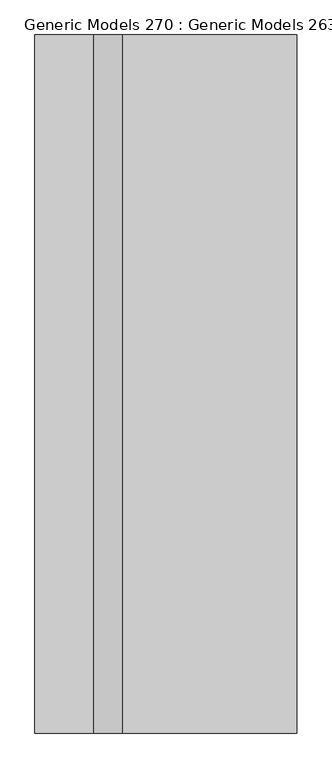
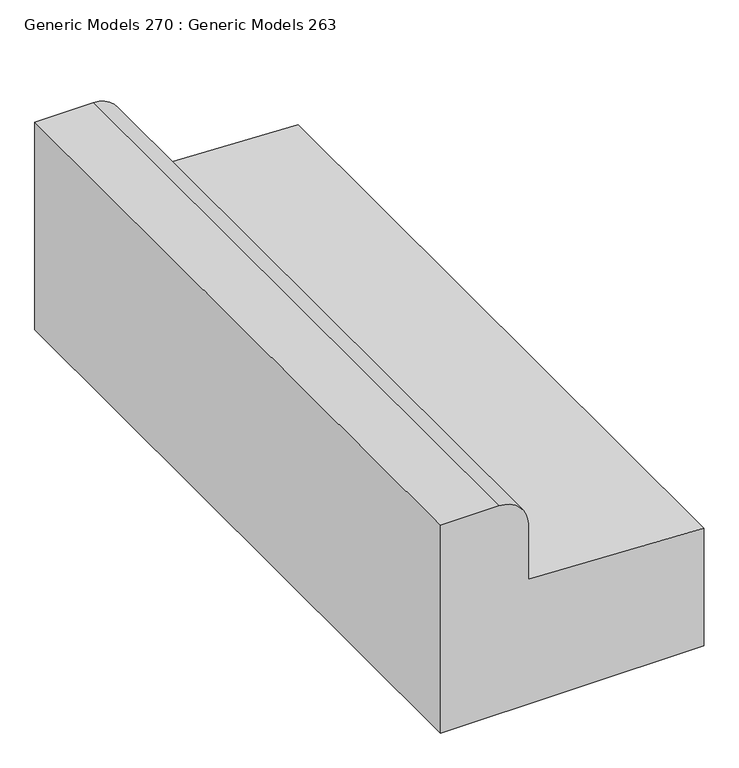
"""IFC4 building model written with IfcOpenShell, lengths in millimetres: proxy geometry, Generic Models 270 : Generic Models 263."""

from ifc_helpers import new_model, si_unit, point, frame, frame_2d, origin, place, context, project, spatial, polyline, circle_curve, trimmed, segment, composite_curve, outline, extrude, source, transform, mapped, element, save


def generic_models_270_generic_models_263_c5a2dacb(model_context):
    return source(origin(), model_context, "Body", "SweptSolid", [
        extrude(outline(composite_curve([segment(polyline([(0.0, 62420.7797726), (0.0, 62319.1797726), (-381.0, 62319.1797726), (-381.0, 62776.3797726), (-165.1, 62776.3797726), (-152.4, 62471.5797726), (-50.8, 62471.5797726)]), True, "CONTINUOUS"), segment(trimmed(circle_curve(frame_2d((-50.8, 62420.7797726)), 50.8), [point((-50.8, 62471.5797726))], [point((0.0, 62420.7797726))], False, "CARTESIAN"), True, "CONTINUOUS")], self_intersect=False)), frame((0.0, -94.4486541, 0.0), z_axis=(0.0, 1.0, 0.0), x_axis=(0.0, 0.0, 1.0)), (0.0, 0.0, 1.0), 1219.2),
    ])


if __name__ == "__main__":
    model = new_model("IFC4")
    model_context = context("Model", 3, world=origin())
    ifc_project = project(units=[si_unit("LENGTHUNIT", "METRE", prefix="MILLI")], contexts=[model_context])
    site = spatial("IfcSite", under=ifc_project)
    building = spatial("IfcBuilding", under=site)
    placement = place(None, origin())
    generic_models_270_generic_models_263_shape = generic_models_270_generic_models_263_c5a2dacb(model_context)
    element("IfcBuildingElementProxy", 1, Name="Generic Models 270 : Generic Models 263", ObjectType="Generic Models 270 : Generic Models 263", at=placement, inside=building, context=model_context, shape_type="MappedRepresentation", body=[
        mapped(generic_models_270_generic_models_263_shape, transform((0.0, 0.0, 0.0), x_axis=(1.0, 0.0, 0.0), y_axis=(0.0, 1.0, 0.0), z_axis=(0.0, 0.0, 1.0))),
    ])
    save(model, "model.ifc")

# Revit data of these elements
# Element 1 (IfcBuildingElementProxy, "Generic Models 270 : Generic Models 263")
#   Materials on its faces: "CONCRETE CURB"
# Materials
#   "CONCRETE CURB": class "Concrete", colour RGB 191 191 191, transparency 0, Description = "Cast-in-place concrete", Cost = 0
